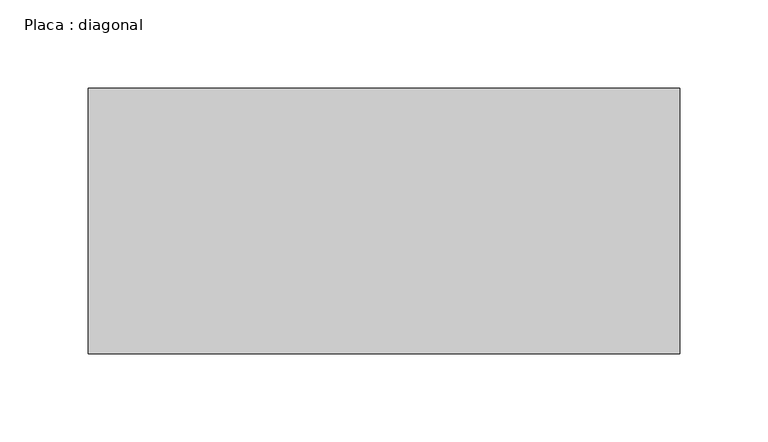
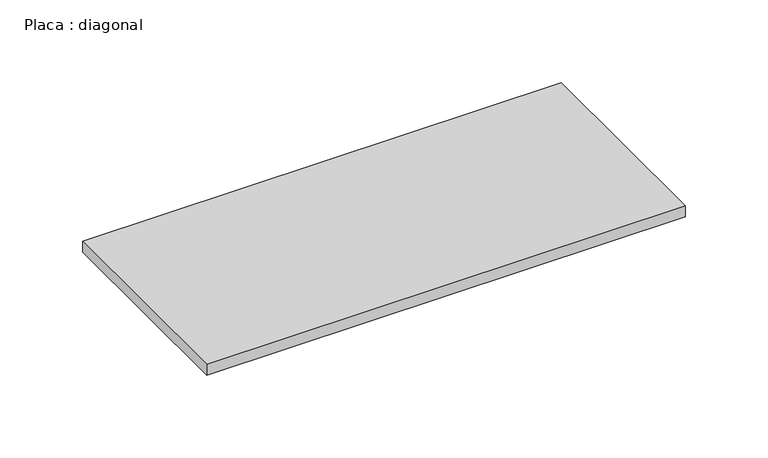
"""IFC4 building model written with IfcOpenShell, lengths in millimetres: beam geometry, Placa : diagonal."""

from ifc_helpers import new_model, si_unit, frame, origin, place, context, project, spatial, polyline, outline, extrude, source, transform, mapped, element, save


def placa_diagonal_780d3588(model_context):
    return source(origin(), model_context, "Body", "SweptSolid", [
        extrude(outline(polyline([(167.4240168, 75.0), (167.4240168, -75.0), (-167.0675395, -75.0), (-167.0675395, 75.0), (167.4240168, 75.0)])), frame((0.0, 0.0, -4.0), z_axis=(0.0, 0.0, 1.0), x_axis=(1.0, 0.0, 0.0)), (0.0, 0.0, 1.0), 8.0),
    ])


if __name__ == "__main__":
    model = new_model("IFC4")
    model_context = context("Model", 3, world=origin())
    ifc_project = project(units=[si_unit("LENGTHUNIT", "METRE", prefix="MILLI")], contexts=[model_context])
    site = spatial("IfcSite", under=ifc_project)
    building = spatial("IfcBuilding", under=site)
    placement = place(None, origin())
    placa_diagonal_shape = placa_diagonal_780d3588(model_context)
    element("IfcBeam", 1, ObjectType="Placa : diagonal", at=placement, inside=building, context=model_context, shape_type="MappedRepresentation", body=[
        mapped(placa_diagonal_shape, transform((0.0, 0.0, 0.0), x_axis=(1.0, 0.0, 0.0), y_axis=(0.0, 1.0, 0.0), z_axis=(0.0, 0.0, 1.0))),
    ])
    save(model, "model.ifc")

# Revit data of these elements
# Type "Placa : diagonal"
#   W = 0
#   Length [instance default] = 1.50 m
#   b = 0.15 m
#   d = 0.008 m
#   A = 0 m²
#   Structural Material [instance default] = Aço, 45-345
# Element 1 (IfcBeam, "Placa : diagonal")
#   Materials on its faces: "Aço, 45-345"
# Materials
#   "Aço, 45-345": class "Metal", colour RGB 247 247 247, transparency 0, Description = "Aço 345 MPa", Cost = 0
